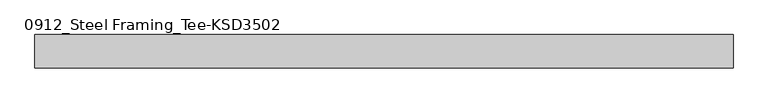
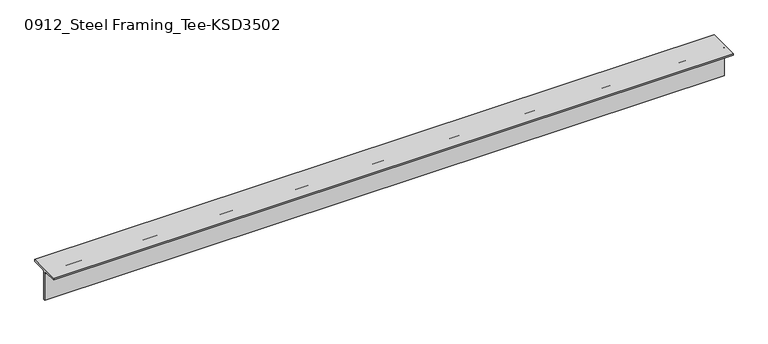
"""IFC4 building model written with IfcOpenShell, lengths in millimetres: member geometry, 0912_Steel Framing_Tee-KSD3502 : H_SB_ASB_CT-150x150x6.5x9."""

from ifc_helpers import new_model, si_unit, point, frame, frame_2d, origin, place, context, project, spatial, polyline, circle_curve, trimmed, segment, composite_curve, outline, extrude, source, transform, mapped, element, save


def member_0912_steel_framing_tee_ksd3502_afed7d49(model_context):
    return source(origin(), model_context, "Body", "SweptSolid", [
        extrude(outline(composite_curve([segment(polyline([(-75.0, 75.0), (75.0, 75.0), (75.0, 66.0), (16.25, 66.0)]), True, "CONTINUOUS"), segment(trimmed(circle_curve(frame_2d((16.25, 53.0)), 13.0), [point((16.25, 66.0))], [point((3.25, 53.0))], True, "CARTESIAN"), True, "CONTINUOUS"), segment(polyline([(3.25, 53.0), (3.25, -75.0), (-3.25, -75.0), (-3.25, 53.0)]), True, "CONTINUOUS"), segment(trimmed(circle_curve(frame_2d((-16.25, 53.0)), 13.0), [point((-3.25, 53.0))], [point((-16.25, 66.0))], True, "CARTESIAN"), True, "CONTINUOUS"), segment(polyline([(-16.25, 66.0), (-75.0, 66.0), (-75.0, 75.0)]), True, "CONTINUOUS")], self_intersect=False)), frame((-1634.1, 0.0, 0.0), z_axis=(1.0, 0.0, 0.0), x_axis=(0.0, 1.0, 0.0)), (0.0, 0.0, 1.0), 3121.7),
    ])


if __name__ == "__main__":
    model = new_model("IFC4")
    model_context = context("Model", 3, world=origin())
    ifc_project = project(units=[si_unit("LENGTHUNIT", "METRE", prefix="MILLI")], contexts=[model_context])
    site = spatial("IfcSite", under=ifc_project)
    building = spatial("IfcBuilding", under=site)
    placement = place(None, origin())
    member_0912_steel_framing_tee_ksd3502_shape = member_0912_steel_framing_tee_ksd3502_afed7d49(model_context)
    element("IfcMember", 1, ObjectType="0912_Steel Framing_Tee-KSD3502 : H_SB_ASB_CT-150x150x6.5x9", at=placement, inside=building, context=model_context, shape_type="MappedRepresentation", body=[
        mapped(member_0912_steel_framing_tee_ksd3502_shape, transform((0.0, 0.0, 0.0), x_axis=(1.0, 0.0, 0.0), y_axis=(0.0, 1.0, 0.0), z_axis=(0.0, 0.0, 1.0))),
    ])
    save(model, "model.ifc")

# Revit data of these elements
# Type "0912_Steel Framing_Tee-KSD3502 : H_SB_ASB_CT-150x150x6.5x9"
#   H_WM Code_1 = "S01AA003-00001 | Main Steel Structure Fabrication Work | Shelter/Building | Light Steel - Standard (30KG/M>Weight) | Material: (   )"
#   H_WM Code_2 = "S03AA029-00001 | Main Steel Structure Erection Work | Shelter/Building | Light Steel (30KG/M>Weight) | Material: (   )"
#   H_WM Code_3 = "S01AA010-00001 | Main Steel Structure Fabrication Work | Shelter/Building | Steel Painting/Coating | for Non-Fireproofed Steel Surface, Surface Preparation, Primer, Second & Final Coat | Material: (   )"
#   H_Q'ty Cal Type Tag = "SB-Q2"
#   Width = 15.0 cm
#   Web Thickness = 0.65 cm
#   Web Fillet = 1.3 cm
#   Section Area = 23.39 cm²
#   Perimeter = 0.60 m²/m
#   Nominal Weight = 18.40 kgf/m
#   Height = 15.0 cm
#   Flange Thickness = 0.9 cm
#   Centroid Vertical = 7.5 cm
#   Centroid Horizontal = 7.5 cm
#   Length [instance default] = 1.5000 m
#   Structural Material [instance default] = Steel, 45-345
#   Warping Constant = (empty or 0)
#   Torsional Moment of Inertia = 0
#   Section Name Key = ""
#   Plastic Modulus weak axis = 0
#   Plastic Modulus strong axis = 0
#   Moment of Inertia weak axis = 0
#   Moment of Inertia strong axis = 0
#   Elastic Modulus weak axis = 0
#   Elastic Modulus strong axis = 0
#   Bolt Spacing = 0
#   Assembly Code = ""
# Element 1 (IfcMember, "0912_Steel Framing_Tee-KSD3502 : H_SB_ASB_CT-150x150x6.5x9")
#   Structural Material = none
# Materials
#   "Steel, 45-345": class "Metal", colour RGB 189 187 185, transparency 0, Description = "Steel 345 MPa", Cost = 0
